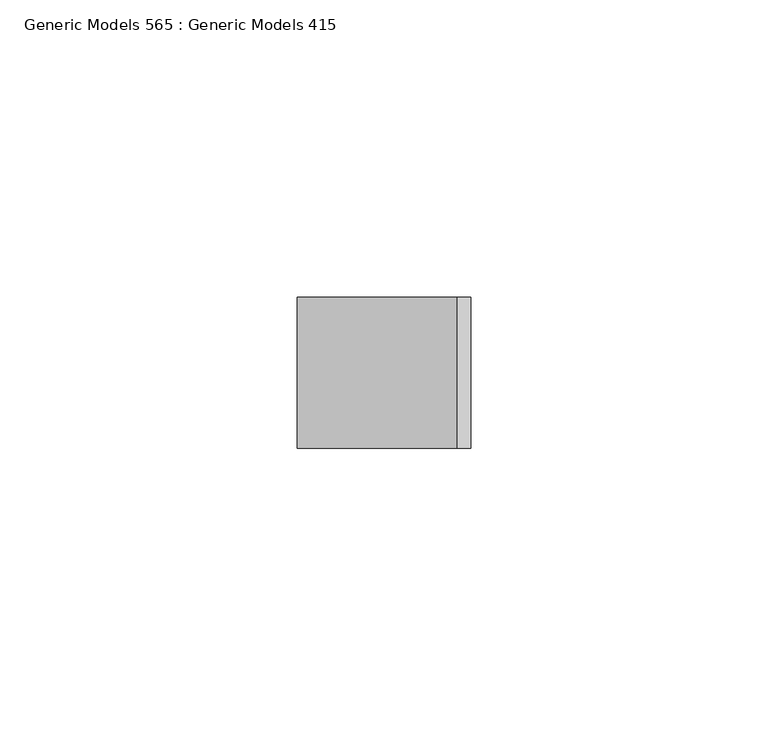
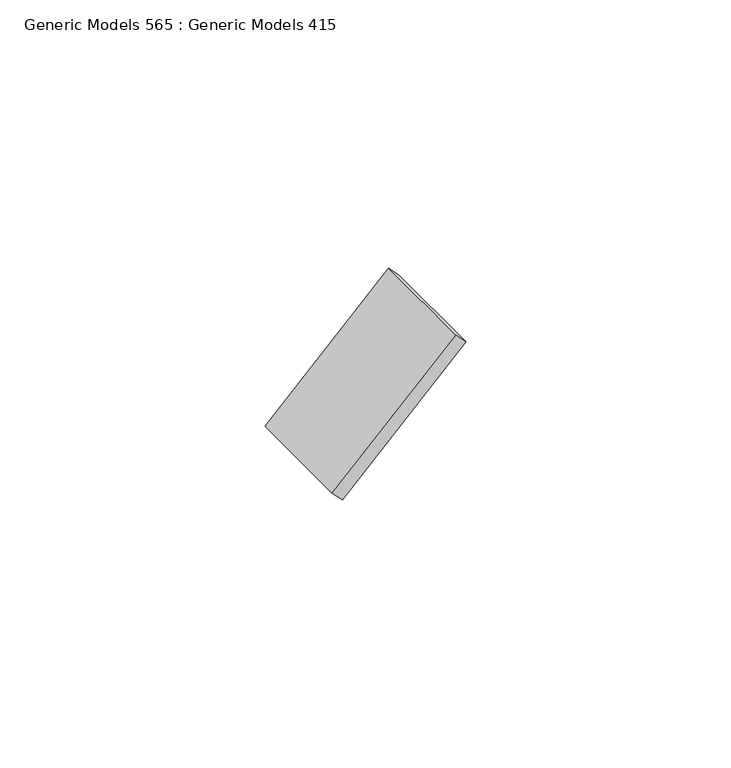
"""IFC4 building model written with IfcOpenShell, lengths in millimetres: proxy geometry, Generic Models 565 : Generic Models 415."""

from ifc_helpers import new_model, si_unit, frame, origin, place, context, project, spatial, polyline, outline, extrude, source, transform, mapped, element, save


def generic_models_565_generic_models_415_2b448b4b(model_context):
    return source(origin(), model_context, "Body", "SweptSolid", [
        extrude(outline(polyline([(0.0, -3.175), (0.0, 0.0), (25.4, 0.0), (25.4, -3.175), (0.0, -3.175)])), frame((7848.0411784, 4501.3863946, 124241.8849742), z_axis=(0.7071067811867181, 0.0, 0.707106781186377), x_axis=(0.0, -1.0, 0.0)), (0.0, 0.0, 1.0), 38.1),
    ])


if __name__ == "__main__":
    model = new_model("IFC4")
    model_context = context("Model", 3, world=origin())
    ifc_project = project(units=[si_unit("LENGTHUNIT", "METRE", prefix="MILLI")], contexts=[model_context])
    site = spatial("IfcSite", under=ifc_project)
    building = spatial("IfcBuilding", under=site)
    placement = place(None, origin())
    generic_models_565_generic_models_415_shape = generic_models_565_generic_models_415_2b448b4b(model_context)
    element("IfcBuildingElementProxy", 1, Name="Generic Models 565 : Generic Models 415", ObjectType="Generic Models 565 : Generic Models 415", at=placement, inside=building, context=model_context, shape_type="MappedRepresentation", body=[
        mapped(generic_models_565_generic_models_415_shape, transform((0.0, 0.0, 0.0), x_axis=(1.0, 0.0, 0.0), y_axis=(0.0, 1.0, 0.0), z_axis=(0.0, 0.0, 1.0))),
    ])
    save(model, "model.ifc")

# Revit data of these elements
# Element 1 (IfcBuildingElementProxy, "Generic Models 565 : Generic Models 415")
#   Materials on its faces: "_WELDED STEEL TABS FOR LOUVER ATTACHMENT"
# Materials
#   "_WELDED STEEL TABS FOR LOUVER ATTACHMENT": class "Metal", colour RGB 199 199 199, transparency 0, Description = "Structural steel 50ksi", Cost = 0
